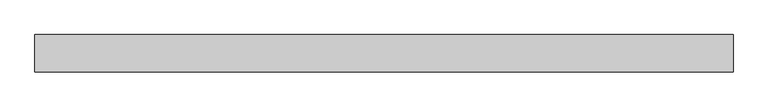
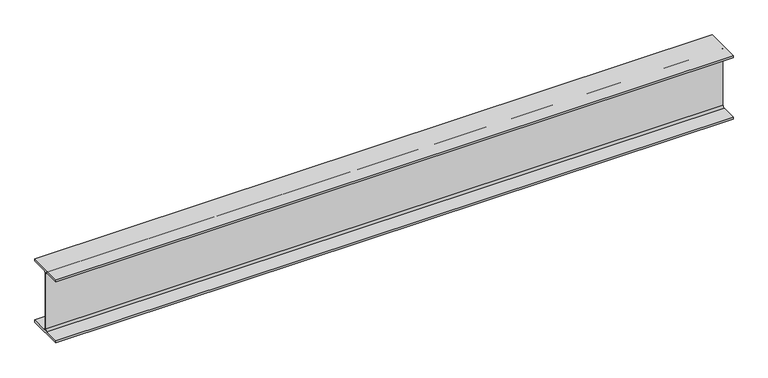
"""IFC4 building model written with IfcOpenShell, lengths in millimetres: beam geometry, Old_Steel Beam_H-KSD3502 : H_SB_ASB_H-200×200x8x12."""

import ifcopenshell
import ifcopenshell.guid

model = None  # the IFC model being written
_history = None  # IfcOwnerHistory: only IFC2X3 demands one
_inside = {}  # id of a spatial element -> (the spatial element, [elements in it])
_under = {}  # id of a project, library or spatial element -> (it, [spatial elements below it])
_declared = {}  # id of a project -> (the project, [libraries it declares])
_typed = {}  # id of a type object -> (the type object, [elements of that type])
_made_of = {}  # id of a material, layer set ... -> (it, [elements and type objects made of it])


def new_model(schema):
    """Start an empty IFC model of exactly this schema.

    Asked for "IFC4X3", IfcOpenShell would pick the latest addendum, in which some entities
    have other attributes; the version numbers below select the first issue.
    IFC2X3 requires an IfcOwnerHistory on every rooted entity: one is made here for all.
    """
    global model, _history
    if schema == "IFC4X3":
        model = ifcopenshell.file(schema_version=(4, 3, 0, 0))
    else:
        model = ifcopenshell.file(schema=schema)
    _inside.clear()
    _under.clear()
    _declared.clear()
    _typed.clear()
    _made_of.clear()
    _history = None
    if model.schema == "IFC2X3":
        org = make("IfcOrganization", Name="unknown")
        user = make(
            "IfcPersonAndOrganization",
            ThePerson=make("IfcPerson", FamilyName="unknown"),
            TheOrganization=org,
        )
        app = make(
            "IfcApplication",
            ApplicationDeveloper=org,
            Version="unknown",
            ApplicationFullName="unknown",
            ApplicationIdentifier="unknown",
        )
        _history = make(
            "IfcOwnerHistory",
            OwningUser=user,
            OwningApplication=app,
            ChangeAction="ADDED",
            CreationDate=0,
        )
    return model


def make(cls, **values):
    """One entity of the class cls with the attributes given. An attribute that is None is left unset."""
    return model.create_entity(
        cls, **{name: value for name, value in values.items() if value is not None}
    )


def rooted(cls, **values):
    """An entity with a GlobalId (a new one), such as an element, a storey or a relation."""
    return make(cls, GlobalId=ifcopenshell.guid.new(), OwnerHistory=_history, **values)


def si_unit(unit_type, name, prefix=None):
    """IfcSIUnit, for example si_unit("LENGTHUNIT", "METRE", prefix="MILLI")."""
    return make("IfcSIUnit", UnitType=unit_type, Prefix=prefix, Name=name)


def assignment(units):
    """IfcUnitAssignment: the units of a project."""
    return None if units is None else make("IfcUnitAssignment", Units=units)


def point(xyz):
    """IfcCartesianPoint."""
    return None if xyz is None else make("IfcCartesianPoint", Coordinates=xyz)


def direction(xyz):
    """IfcDirection."""
    return None if xyz is None else make("IfcDirection", DirectionRatios=xyz)


def frame(location, z_axis=None, x_axis=None):
    """IfcAxis2Placement3D, a coordinate frame: its origin and axes. An axis left out is left unset."""
    return make(
        "IfcAxis2Placement3D",
        Location=point(location),
        Axis=direction(z_axis),
        RefDirection=direction(x_axis),
    )


def frame_2d(location, x_axis=None):
    """IfcAxis2Placement2D, a coordinate frame in the plane: its origin and x axis."""
    return make(
        "IfcAxis2Placement2D", Location=point(location), RefDirection=direction(x_axis)
    )


def origin():
    """The frame at (0, 0, 0) with its axes left unset."""
    return frame((0.0, 0.0, 0.0))


def place(relative_to, where):
    """IfcLocalPlacement: puts the frame where relative to a parent placement (None: the world)."""
    return make(
        "IfcLocalPlacement", PlacementRelTo=relative_to, RelativePlacement=where
    )


def context(
    kind, dimensions, precision=None, world=None, true_north=None, identifier=None
):
    """IfcGeometricRepresentationContext, for example the 3D "Model" context."""
    return make(
        "IfcGeometricRepresentationContext",
        ContextIdentifier=identifier,
        ContextType=kind,
        CoordinateSpaceDimension=dimensions,
        Precision=precision,
        WorldCoordinateSystem=world,
        TrueNorth=true_north,
    )


def project(units=None, contexts=None):
    """IfcProject with its units and contexts."""
    return rooted(
        "IfcProject",
        Name="project",
        RepresentationContexts=contexts,
        UnitsInContext=assignment(units),
    )


def spatial(cls, under=None, at=None, **own):
    """A site, building, storey or space (cls), placed at a placement, below another one or the project."""
    s = rooted(cls, ObjectPlacement=at, **own)
    if under is not None:
        _under.setdefault(under.id(), (under, []))[1].append(s)
    return s


def polyline(points):
    """IfcPolyline through the points."""
    return make("IfcPolyline", Points=[point(p) for p in points])


def circle_curve(where, radius):
    """IfcCircle in the frame where."""
    return make("IfcCircle", Position=where, Radius=radius)


def trimmed(basis, trim1, trim2, sense, master):
    """IfcTrimmedCurve: the piece of a basis curve between two trims."""
    return make(
        "IfcTrimmedCurve",
        BasisCurve=basis,
        Trim1=trim1,
        Trim2=trim2,
        SenseAgreement=sense,
        MasterRepresentation=master,
    )


def segment(curve, same_sense, transition):
    """IfcCompositeCurveSegment."""
    return make(
        "IfcCompositeCurveSegment",
        Transition=transition,
        SameSense=same_sense,
        ParentCurve=curve,
    )


def composite_curve(segments, self_intersect=None):
    """IfcCompositeCurve: segments joined end to end."""
    return make("IfcCompositeCurve", Segments=segments, SelfIntersect=self_intersect)


def outline(outer, holes=None, kind="AREA"):
    """IfcArbitraryClosedProfileDef: a profile drawn as a closed curve; with holes, ...WithVoids."""
    if holes is None:
        return make("IfcArbitraryClosedProfileDef", ProfileType=kind, OuterCurve=outer)
    return make(
        "IfcArbitraryProfileDefWithVoids",
        ProfileType=kind,
        OuterCurve=outer,
        InnerCurves=holes,
    )


def extrude(swept, where, along, depth):
    """IfcExtrudedAreaSolid: the profile swept, set in the frame where, extruded along a direction by depth."""
    return make(
        "IfcExtrudedAreaSolid",
        SweptArea=swept,
        Position=where,
        ExtrudedDirection=direction(along),
        Depth=depth,
    )


def shape(context_of_items, identifier, shape_type, items):
    """IfcShapeRepresentation: the items that make up one representation, for example the "Body"."""
    return make(
        "IfcShapeRepresentation",
        ContextOfItems=context_of_items,
        RepresentationIdentifier=identifier,
        RepresentationType=shape_type,
        Items=items,
    )


def source(mapping_origin, context_of_items, identifier, shape_type, items):
    """IfcRepresentationMap: a shape defined once, which mapped items show again and again."""
    return make(
        "IfcRepresentationMap",
        MappingOrigin=mapping_origin,
        MappedRepresentation=shape(context_of_items, identifier, shape_type, items),
    )


def transform(
    local_origin,
    x_axis=None,
    y_axis=None,
    z_axis=None,
    scale=None,
    scale2=None,
    scale3=None,
    uniform=True,
):
    """IfcCartesianTransformationOperator3D, or its non-uniform kind. x_axis, y_axis, z_axis: its Axis1, 2, 3."""
    if uniform:
        return make(
            "IfcCartesianTransformationOperator3D",
            Axis1=direction(x_axis),
            Axis2=direction(y_axis),
            LocalOrigin=point(local_origin),
            Scale=scale,
            Axis3=direction(z_axis),
        )
    return make(
        "IfcCartesianTransformationOperator3DnonUniform",
        Axis1=direction(x_axis),
        Axis2=direction(y_axis),
        LocalOrigin=point(local_origin),
        Scale=scale,
        Axis3=direction(z_axis),
        Scale2=scale2,
        Scale3=scale3,
    )


def mapped(mapping_source, mapping_target):
    """IfcMappedItem: shows the shape of a source again, moved by a transform."""
    return make(
        "IfcMappedItem", MappingSource=mapping_source, MappingTarget=mapping_target
    )


def made_of(thing, what):
    """Note that an element or type object is made of a material, layer set ...; save() writes the relation."""
    if what is not None:
        _made_of.setdefault(what.id(), (what, []))[1].append(thing)
    return thing


def element(
    cls,
    number,
    at=None,
    inside=None,
    cuts=None,
    type_object=None,
    material=None,
    context=None,
    identifier="Body",
    shape_type=None,
    held_by="IfcProductDefinitionShape",
    body=None,
    shapes=None,
    **own,
):
    """One element of the class cls, such as IfcWall. Its Tag is "e" and its number.

    at: its placement. inside: the storey or other place that contains it. cuts: it is an
    opening in that element (IfcRelVoidsElement). A single representation is given by context,
    identifier, shape_type and body (its items); several are given by shapes. held_by: the class
    of the entity that holds the representations. save() writes the other relations.
    """
    e = rooted(cls, Tag="e%d" % number, ObjectPlacement=at, **own)
    if body is not None:
        shapes = [shape(context, identifier, shape_type, body)]
    if shapes is not None:
        e.Representation = make(held_by, Representations=shapes)
    if inside is not None:
        _inside.setdefault(inside.id(), (inside, []))[1].append(e)
    if cuts is not None:
        rooted(
            "IfcRelVoidsElement", RelatingBuildingElement=cuts, RelatedOpeningElement=e
        )
    if type_object is not None:
        _typed.setdefault(type_object.id(), (type_object, []))[1].append(e)
    return made_of(e, material)


def aggregate(whole, parts):
    """IfcRelAggregates: a whole, such as a stair, and the parts it consists of."""
    return rooted("IfcRelAggregates", RelatingObject=whole, RelatedObjects=parts)


def save(model, path):
    """Write the relations noted so far, then the file.

    IfcRelAggregates (storeys below a building ...), IfcRelContainedInSpatialStructure (elements
    in a storey), IfcRelDefinesByType, IfcRelAssociatesMaterial and IfcRelDeclares: one each for
    every whole, place, type object, material and project.
    """
    for whole, parts in _under.values():
        aggregate(whole, parts)
    for where, things in _inside.values():
        rooted(
            "IfcRelContainedInSpatialStructure",
            RelatedElements=things,
            RelatingStructure=where,
        )
    for kind, things in _typed.values():
        rooted("IfcRelDefinesByType", RelatedObjects=things, RelatingType=kind)
    for what, things in _made_of.values():
        rooted("IfcRelAssociatesMaterial", RelatedObjects=things, RelatingMaterial=what)
    for by, libraries in _declared.values():
        rooted("IfcRelDeclares", RelatingContext=by, RelatedDefinitions=libraries)
    model.write(path)


def beam_2c81aa5d(model_context):
    return source(origin(), model_context, "Body", "SweptSolid", [
        extrude(outline(composite_curve([segment(polyline([(82.5, -141.5), (82.5, -151.7), (-82.5, -151.7), (-82.5, -141.5), (-11.9, -141.5)]), True, "CONTINUOUS"), segment(trimmed(circle_curve(frame_2d((-11.9, -132.6)), 8.9), [point((-11.9, -141.5))], [point((-3.0, -132.6))], True, "CARTESIAN"), True, "CONTINUOUS"), segment(polyline([(-3.0, -132.6), (-3.0, 132.6)]), True, "CONTINUOUS"), segment(trimmed(circle_curve(frame_2d((-11.9, 132.6)), 8.9), [point((-3.0, 132.6))], [point((-11.9, 141.5))], True, "CARTESIAN"), True, "CONTINUOUS"), segment(polyline([(-11.9, 141.5), (-82.5, 141.5), (-82.5, 151.7), (82.5, 151.7), (82.5, 141.5), (11.9, 141.5)]), True, "CONTINUOUS"), segment(trimmed(circle_curve(frame_2d((11.9, 132.6)), 8.9), [point((11.9, 141.5))], [point((3.0, 132.6))], True, "CARTESIAN"), True, "CONTINUOUS"), segment(polyline([(3.0, 132.6), (3.0, -132.6)]), True, "CONTINUOUS"), segment(trimmed(circle_curve(frame_2d((11.9, -132.6)), 8.9), [point((3.0, -132.6))], [point((11.9, -141.5))], True, "CARTESIAN"), True, "CONTINUOUS"), segment(polyline([(11.9, -141.5), (82.5, -141.5)]), True, "CONTINUOUS")], self_intersect=False)), frame((-1489.1986147, 0.0, 0.0), z_axis=(1.0, 0.0, 0.0), x_axis=(0.0, 1.0, 0.0)), (0.0, 0.0, 1.0), 3067.173634),
    ])


if __name__ == "__main__":
    model = new_model("IFC4")
    model_context = context("Model", 3, world=origin())
    ifc_project = project(units=[si_unit("LENGTHUNIT", "METRE", prefix="MILLI")], contexts=[model_context])
    site = spatial("IfcSite", under=ifc_project)
    building = spatial("IfcBuilding", under=site)
    placement = place(None, origin())
    beam_shape = beam_2c81aa5d(model_context)
    element("IfcBeam", 1, ObjectType="Old_Steel Beam_H-KSD3502 : H_SB_ASB_H-200×200x8x12", at=placement, inside=building, context=model_context, shape_type="MappedRepresentation", body=[
        mapped(beam_shape, transform((0.0, 0.0, 0.0), x_axis=(1.0, 0.0, 0.0), y_axis=(0.0, 1.0, 0.0), z_axis=(0.0, 0.0, 1.0))),
    ])
    save(model, "model.ifc")

# Revit data of these elements
# Type "Old_Steel Beam_H-KSD3502 : H_SB_ASB_H-200×200x8x12"
#   Width = 20.0 cm
#   Web Thickness = 0.8 cm
#   Web Fillet = 1.3 cm
#   Warping Constant = 141376.0 cm⁶
#   Torsional Moment of Inertia = 26.2485 cm⁴
#   Torsional Modulus = 1.0 cm³
#   Section Area = 63.53 cm²
#   Plastic Modulus weak axis = 244.0 cm³
#   Plastic Modulus strong axis = 525.0 cm³
#   Perimeter = 1.16 m²/m
#   Nominal Weight = 49.90 kgf/m
#   Moment of Inertia weak axis = 1600.00 cm⁴
#   Moment of Inertia strong axis = 4720.00 cm⁴
#   Height = 20.0 cm
#   Flange Thickness = 1.2 cm
#   Elastic Modulus weak axis = 160.0 cm³
#   Elastic Modulus strong axis = 472.0 cm³
#   Centroid Vertical = 10.0 cm
#   Centroid Horizontal = 10.0 cm
#   Length [instance default] = 1.5240 m
#   Structural Material [instance default] = Steel, 45-345
#   Assembly Code = ""
# Element 1 (IfcBeam, "Old_Steel Beam_H-KSD3502 : H_SB_ASB_H-200×200x8x12")
#   Structural Material = none
# Materials
#   "Steel, 45-345": class "Metal", colour RGB 189 187 185, transparency 0, Description = "Steel 345 MPa", Cost = 0
